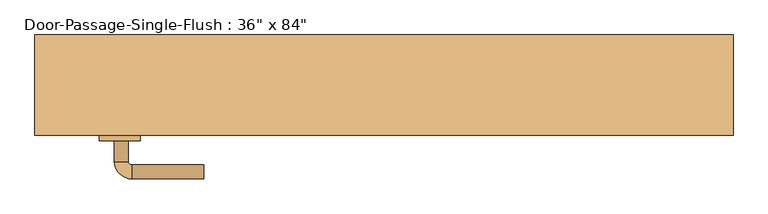
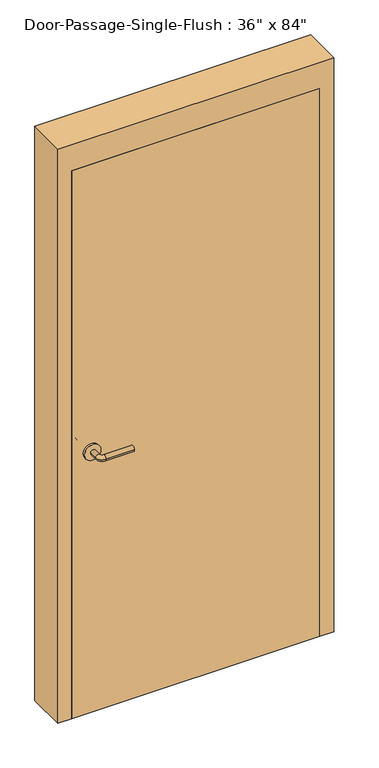
"""IFC4 building model written with IfcOpenShell, lengths in millimetres: door geometry."""

from ifc_helpers import new_model, si_unit, point, frame, frame_2d, origin, origin_with_axes, place, context, project, spatial, polyline, circle_curve, ellipse_curve, trimmed, segment, composite_curve, outline, extrude, faceted_brep, source, transform, mapped, element, save
from ifc_brep_helpers import plane_surface, cylinder_surface, revolved_surface, advanced_brep


def door_fea31935(model_context):
    return source(origin(), model_context, "Body", "SolidModel", [
        advanced_brep(
        [(-392.190625, -180.9125, 1016.0), (-372.190625, -180.9125, 1016.0), (-392.190625, -150.9125, 1016.0), (-372.190625, -150.9125, 1016.0), (-367.190625, -145.9125, 1016.0), (-367.190625, -125.9125, 1016.0), (-262.190625, -125.9125, 1016.0), (-262.190625, -145.9125, 1016.0)],
        [
            (0, 1, circle_curve(frame((-382.190625, -180.9125, 1016.0), z_axis=(0.0, -1.0, 0.0), x_axis=(1.0, 0.0, 0.0)), 10.0)),
            (1, 0, circle_curve(frame((-382.190625, -180.9125, 1016.0), z_axis=(0.0, -1.0, 0.0), x_axis=(1.0, 0.0, 0.0)), 10.0)),
            (0, 2),
            (2, 3, circle_curve(frame((-382.190625, -150.9125, 1016.0), z_axis=(0.0, -1.0, 0.0), x_axis=(1.0, 0.0, 0.0)), 10.0)),
            (3, 1),
            (3, 2, circle_curve(frame((-382.190625, -150.9125, 1016.0), z_axis=(0.0, -1.0, 0.0), x_axis=(1.0, 0.0, 0.0)), 10.0)),
            (4, 3, circle_curve(frame((-367.190625, -150.9125, 1016.0), z_axis=(0.0, 0.0, 1.0), x_axis=(-1.0, 0.0, 0.0)), 5.0)),
            (2, 5, circle_curve(frame((-367.190625, -150.9125, 1016.0), z_axis=(0.0, 0.0, -1.0), x_axis=(-1.0, 0.0, 0.0)), 25.0)),
            (5, 4, circle_curve(frame((-367.190625, -135.9125, 1016.0), z_axis=(-1.0, 0.0, 0.0), x_axis=(0.0, -1.0, 0.0)), 10.0)),
            (4, 5, circle_curve(frame((-367.190625, -135.9125, 1016.0), z_axis=(-1.0, 0.0, 0.0), x_axis=(0.0, -1.0, 0.0)), 10.0)),
            (6, 7, circle_curve(frame((-262.190625, -135.9125, 1016.0), z_axis=(1.0, 0.0, 0.0), x_axis=(0.0, -1.0, 0.0)), 10.0)),
            (7, 6, circle_curve(frame((-262.190625, -135.9125, 1016.0), z_axis=(1.0, 0.0, 0.0), x_axis=(0.0, -1.0, 0.0)), 10.0)),
            (5, 6),
            (7, 4),
        ],
        [
            plane_surface(frame((-382.190625, -180.9125, 1016.0), z_axis=(0.0, -1.0, 0.0), x_axis=(0.0, 0.0, 1.0))),
            cylinder_surface(frame((-382.190625, -180.9125, 1016.0), z_axis=(0.0, -1.0, 0.0), x_axis=(1.0, 0.0, 0.0)), 10.0),
            revolved_surface(trimmed(ellipse_curve(frame((-382.190625, -150.9125, 1016.0), z_axis=(0.0, -1.0, 0.0), x_axis=(1.0, 0.0, 0.0)), 10.0, 10.0), [point((-392.190625, -150.9125, 1016.0))], [point((-372.190625, -150.9125, 1016.0))], True, "CARTESIAN"), (-367.190625, -150.9125, 1016.0), (0.0, 0.0, -1.0)),
            revolved_surface(trimmed(ellipse_curve(frame((-382.190625, -150.9125, 1016.0), z_axis=(0.0, -1.0, 0.0), x_axis=(1.0, 0.0, 0.0)), 10.0, 10.0), [point((-372.190625, -150.9125, 1016.0))], [point((-392.190625, -150.9125, 1016.0))], True, "CARTESIAN"), (-367.190625, -150.9125, 1016.0), (0.0, 0.0, -1.0)),
            plane_surface(frame((-262.190625, -135.9125, 1016.0), z_axis=(1.0, 0.0, 0.0), x_axis=(0.0, 0.0, 1.0))),
            cylinder_surface(frame((-367.190625, -135.9125, 1016.0), z_axis=(-1.0, 0.0, 0.0), x_axis=(0.0, -1.0, 0.0)), 10.0),
        ],
        [
            (0, [[1, 2]]),
            (1, [[-1, 3, 4, 5]]),
            (1, [[-2, -5, 6, -3]]),
            (2, [[7, -4, 8, 9]]),
            (3, [[-8, -6, -7, 10]]),
            (4, [[11, 12]]),
            (5, [[-9, 13, -12, 14]]),
            (5, [[-10, -14, -11, -13]]),
        ],
    ),
        extrude(outline(composite_curve([segment(trimmed(circle_curve(frame_2d((1016.0, -384.690625)), 30.0), [point((1016.0, -414.690625))], [point((1016.0, -354.690625))], False, "CARTESIAN"), True, "CONTINUOUS"), segment(trimmed(circle_curve(frame_2d((1016.0, -384.690625)), 30.0), [point((1016.0, -354.690625))], [point((1016.0, -414.690625))], False, "CARTESIAN"), True, "CONTINUOUS")], self_intersect=False)), frame((0.0, -188.9125, 0.0), z_axis=(0.0, 1.0, 0.0), x_axis=(0.0, 0.0, 1.0)), (0.0, 0.0, 1.0), 8.0),
        advanced_brep(
        [(-392.190625, -241.3625, 1016.0), (-372.190625, -241.3625, 1016.0), (-372.190625, -271.3625, 1016.0), (-392.190625, -271.3625, 1016.0), (-367.190625, -276.3625, 1016.0), (-367.190625, -296.3625, 1016.0), (-262.190625, -296.3625, 1016.0), (-262.190625, -276.3625, 1016.0)],
        [
            (0, 1, circle_curve(frame((-382.190625, -241.3625, 1016.0), z_axis=(0.0, 1.0, 0.0), x_axis=(1.0, 0.0, 0.0)), 10.0)),
            (1, 0, circle_curve(frame((-382.190625, -241.3625, 1016.0), z_axis=(0.0, 1.0, 0.0), x_axis=(1.0, 0.0, 0.0)), 10.0)),
            (1, 2),
            (2, 3, circle_curve(frame((-382.190625, -271.3625, 1016.0), z_axis=(0.0, 1.0, 0.0), x_axis=(1.0, 0.0, 0.0)), 10.0)),
            (3, 0),
            (3, 2, circle_curve(frame((-382.190625, -271.3625, 1016.0), z_axis=(0.0, 1.0, 0.0), x_axis=(1.0, 0.0, 0.0)), 10.0)),
            (4, 5, circle_curve(frame((-367.190625, -286.3625, 1016.0), z_axis=(-1.0, 0.0, 0.0), x_axis=(0.0, 1.0, 0.0)), 10.0)),
            (5, 3, circle_curve(frame((-367.190625, -271.3625, 1016.0), z_axis=(0.0, 0.0, -1.0), x_axis=(-1.0, 0.0, 0.0)), 25.0)),
            (2, 4, circle_curve(frame((-367.190625, -271.3625, 1016.0), z_axis=(0.0, 0.0, 1.0), x_axis=(-1.0, 0.0, 0.0)), 5.0)),
            (5, 4, circle_curve(frame((-367.190625, -286.3625, 1016.0), z_axis=(-1.0, 0.0, 0.0), x_axis=(0.0, 1.0, 0.0)), 10.0)),
            (6, 7, circle_curve(frame((-262.190625, -286.3625, 1016.0), z_axis=(1.0, 0.0, 0.0), x_axis=(0.0, 1.0, 0.0)), 10.0)),
            (7, 6, circle_curve(frame((-262.190625, -286.3625, 1016.0), z_axis=(1.0, 0.0, 0.0), x_axis=(0.0, 1.0, 0.0)), 10.0)),
            (4, 7),
            (6, 5),
        ],
        [
            plane_surface(frame((-382.190625, -241.3625, 1016.0), z_axis=(0.0, 1.0, 0.0), x_axis=(0.0, 0.0, 1.0))),
            cylinder_surface(frame((-382.190625, -241.3625, 1016.0), z_axis=(0.0, 1.0, 0.0), x_axis=(1.0, 0.0, 0.0)), 10.0),
            revolved_surface(trimmed(ellipse_curve(frame((-382.190625, -271.3625, 1016.0), z_axis=(0.0, -1.0, 0.0), x_axis=(1.0, 0.0, 0.0)), 10.0, 10.0), [point((-392.190625, -271.3625, 1016.0))], [point((-372.190625, -271.3625, 1016.0))], True, "CARTESIAN"), (-367.190625, -271.3625, 1016.0), (0.0, 0.0, -1.0)),
            revolved_surface(trimmed(ellipse_curve(frame((-382.190625, -271.3625, 1016.0), z_axis=(0.0, -1.0, 0.0), x_axis=(1.0, 0.0, 0.0)), 10.0, 10.0), [point((-372.190625, -271.3625, 1016.0))], [point((-392.190625, -271.3625, 1016.0))], True, "CARTESIAN"), (-367.190625, -271.3625, 1016.0), (0.0, 0.0, -1.0)),
            plane_surface(frame((-262.190625, -286.3625, 1016.0), z_axis=(1.0, 0.0, 0.0), x_axis=(0.0, 0.0, 1.0))),
            cylinder_surface(frame((-367.190625, -286.3625, 1016.0), z_axis=(-1.0, 0.0, 0.0), x_axis=(0.0, 1.0, 0.0)), 10.0),
        ],
        [
            (0, [[1, 2]]),
            (1, [[3, 4, 5, -2]]),
            (1, [[-5, 6, -3, -1]]),
            (2, [[7, 8, -4, 9]]),
            (3, [[10, -9, -6, -8]]),
            (4, [[11, 12]]),
            (5, [[13, -11, 14, -7]]),
            (5, [[-14, -12, -13, -10]]),
        ],
    ),
        extrude(outline(composite_curve([segment(trimmed(circle_curve(frame_2d((1016.0, -384.690625)), 30.0), [point((1016.0, -414.690625))], [point((1016.0, -354.690625))], False, "CARTESIAN"), True, "CONTINUOUS"), segment(trimmed(circle_curve(frame_2d((1016.0, -384.690625)), 30.0), [point((1016.0, -354.690625))], [point((1016.0, -414.690625))], False, "CARTESIAN"), True, "CONTINUOUS")], self_intersect=False)), frame((0.0, -241.3625, 0.0), z_axis=(0.0, 1.0, 0.0), x_axis=(0.0, 0.0, 1.0)), (0.0, 0.0, 1.0), 8.0),
        faceted_brep([(457.2, -184.15, 0.0), (441.325, -184.15, 0.0), (441.325, -136.525, 0.0), (457.2, -136.525, 0.0), (457.2, -87.3125, 0.0), (508.0, -87.3125, 0.0), (508.0, -233.3625, 0.0), (457.2, -233.3625, 0.0), (457.2, -233.3625, 2133.6), (457.2, -184.15, 2133.6), (508.0, -233.3625, 2235.2), (-508.0, -233.3625, 2235.2), (-508.0, -233.3625, 0.0), (-457.2, -233.3625, 0.0), (-457.2, -233.3625, 2133.6), (508.0, -87.3125, 2235.2), (457.2, -87.3125, 2133.6), (-457.2, -87.3125, 2133.6), (-457.2, -87.3125, 0.0), (-508.0, -87.3125, 0.0), (-508.0, -87.3125, 2235.2), (457.2, -136.525, 2133.6), (441.325, -136.525, 2117.725), (-441.325, -136.525, 2117.725), (-441.325, -136.525, 0.0), (-457.2, -136.525, 0.0), (-457.2, -136.525, 2133.6), (441.325, -184.15, 2117.725), (-457.2, -184.15, 2133.6), (-457.2, -184.15, 0.0), (-441.325, -184.15, 0.0), (-441.325, -184.15, 2117.725)], [[[0, 1, 2, 3, 4, 5, 6, 7]], [[7, 8, 9, 0]], [[6, 10, 11, 12, 13, 14, 8, 7]], [[5, 15, 10, 6]], [[4, 16, 17, 18, 19, 20, 15, 5]], [[3, 21, 16, 4]], [[2, 22, 23, 24, 25, 26, 21, 3]], [[1, 27, 22, 2]], [[0, 9, 28, 29, 30, 31, 27, 1]], [[8, 14, 28, 9]], [[16, 21, 26, 17]], [[22, 27, 31, 23]], [[12, 19, 18, 25, 24, 30, 29, 13]], [[13, 29, 28, 14]], [[11, 20, 19, 12]], [[17, 26, 25, 18]], [[23, 31, 30, 24]], [[15, 20, 11, 10]]]),
        extrude(outline(polyline([(457.2, -188.9125), (457.2, -233.3625), (-457.2, -233.3625), (-457.2, -188.9125), (457.2, -188.9125)])), origin_with_axes(), (0.0, 0.0, 1.0), 2133.6),
    ])


if __name__ == "__main__":
    model = new_model("IFC4")
    model_context = context("Model", 3, world=origin())
    ifc_project = project(units=[si_unit("LENGTHUNIT", "METRE", prefix="MILLI")], contexts=[model_context])
    site = spatial("IfcSite", under=ifc_project)
    building = spatial("IfcBuilding", under=site)
    placement = place(None, origin())
    door_shape = door_fea31935(model_context)
    element("IfcDoor", 1, ObjectType="Door-Passage-Single-Flush : 36\" x 84\"", at=placement, inside=building, context=model_context, shape_type="MappedRepresentation", body=[
        mapped(door_shape, transform((0.0, 0.0, 0.0), x_axis=(1.0, 0.0, 0.0), y_axis=(0.0, 1.0, 0.0), z_axis=(0.0, 0.0, 1.0))),
    ])
    save(model, "model.ifc")

# Revit data of these elements
# Type "Door-Passage-Single-Flush : 36\" x 84\""
#   Type Mark = "35"
#   Assembly Code = "B2030200"
#   Analytic Construction = "Wooden"
#   Thickness = 0' - 1 3/4"
#   Thermal Resistance (R) = 2.5876 (h·ft²·°F)/BTU
#   Swing Angle [instance default] = 90.00°
#   Strike Height = 3' - 4"
#   Rough Width [instance default] = 3' - 4"
#   Rough Height [instance default] = 7' - 4"
#   MF Opening Height [instance default] = 0' - 4"
#   MF Opening Width [instance default] = 0' - 4"
#   Inset Calculate [instance default] = 0' - 4"
#   Masonry Inset [instance default] = 0' - 1"
#   Height = 7' - 0"
#   Width = 3' - 0"
#   Heat Transfer Coefficient (U) = 0.3865 BTU/(h·ft²·°F)
#   Masonry Frame Depth = 0' - 5 3/4"
#   Masonry Frame [instance default] = yes
#   Function = 1
#   Dry Wall Frame [instance default] = no
#   Panel Material = Wood - Birch
#   Frame Material = Metal - Paint Finish - Grey
#   Door Handle Material = Aluminum
#   Visual Light Transmittance = 0
#   Solar Heat Gain Coefficient = 0
#   Wall Closure = (empty or 0)
# Element 1 (IfcDoor, "Door-Passage-Single-Flush : 36\" x 84\"")
#   Inset Calculate = 0' - 3"
#   Masonry Inset = 0' - 0"
#   Materials on its faces: "Aluminum", "Metal - Paint Finish - Grey", "Wood - Birch"
# Materials
#   "Wood - Birch": class "Wood", colour RGB 166 116 52, transparency 0, Cost = 0
#   "Metal - Paint Finish - Grey": class "Paint", colour RGB 104 104 104, transparency 0, Cost = 0
#   "Aluminum": class "Metal", colour RGB 247 247 247, transparency 0, Description = "Aluminum 6061", Cost = 0
